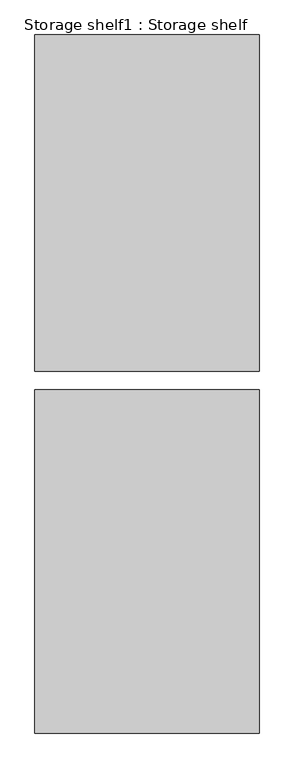
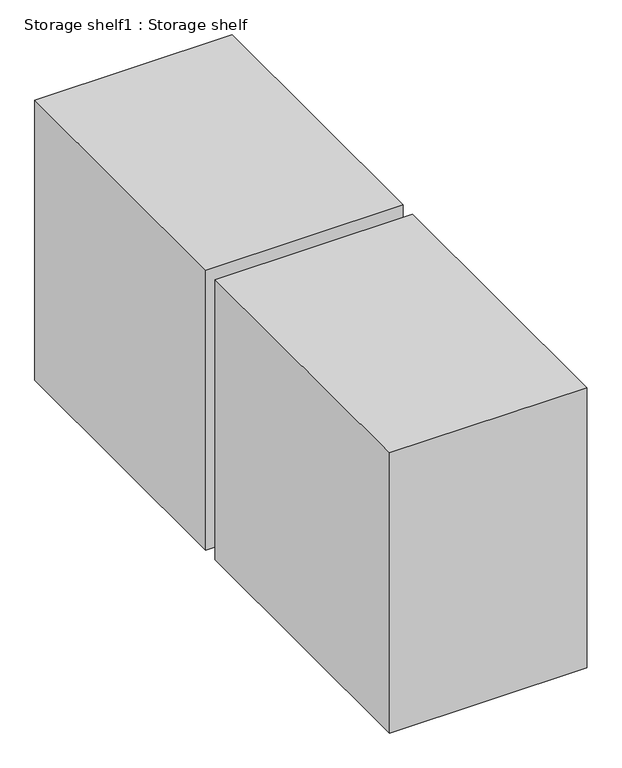
"""IFC4 building model written with IfcOpenShell, lengths in millimetres: furniture geometry, Storage shelf1 : Storage shelf."""

from ifc_helpers import new_model, si_unit, origin, origin_with_axes, place, context, project, spatial, polyline, outline, extrude, source, transform, mapped, element, save


def storage_shelf1_storage_shelf_b77c188d(model_context):
    return source(origin(), model_context, "Body", "SweptSolid", [
        extrude(outline(polyline([(28842.4870052, 7913.3615366), (28232.8870052, 7913.3615366), (28232.8870052, 8827.7615366), (28842.4870052, 8827.7615366), (28842.4870052, 7913.3615366)])), origin_with_axes(), (0.0, 0.0, 1.0), 914.4),
        extrude(outline(polyline([(28842.4870052, 6928.9043874), (28232.8870052, 6928.9043874), (28232.8870052, 7862.5615366), (28842.4870052, 7862.5615366), (28842.4870052, 6928.9043874)])), origin_with_axes(), (0.0, 0.0, 1.0), 914.4),
    ])


if __name__ == "__main__":
    model = new_model("IFC4")
    model_context = context("Model", 3, world=origin())
    ifc_project = project(units=[si_unit("LENGTHUNIT", "METRE", prefix="MILLI")], contexts=[model_context])
    site = spatial("IfcSite", under=ifc_project)
    building = spatial("IfcBuilding", under=site)
    placement = place(None, origin())
    storage_shelf1_storage_shelf_shape = storage_shelf1_storage_shelf_b77c188d(model_context)
    element("IfcFurniture", 1, ObjectType="Storage shelf1 : Storage shelf", at=placement, inside=building, context=model_context, shape_type="MappedRepresentation", body=[
        mapped(storage_shelf1_storage_shelf_shape, transform((0.0, 0.0, 0.0), x_axis=(1.0, 0.0, 0.0), y_axis=(0.0, 1.0, 0.0), z_axis=(0.0, 0.0, 1.0))),
    ])
    save(model, "model.ifc")
